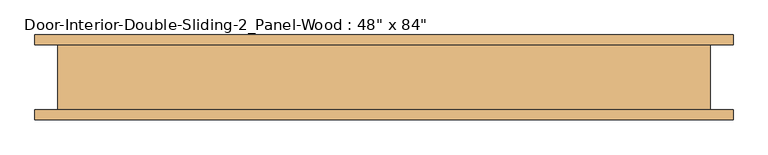
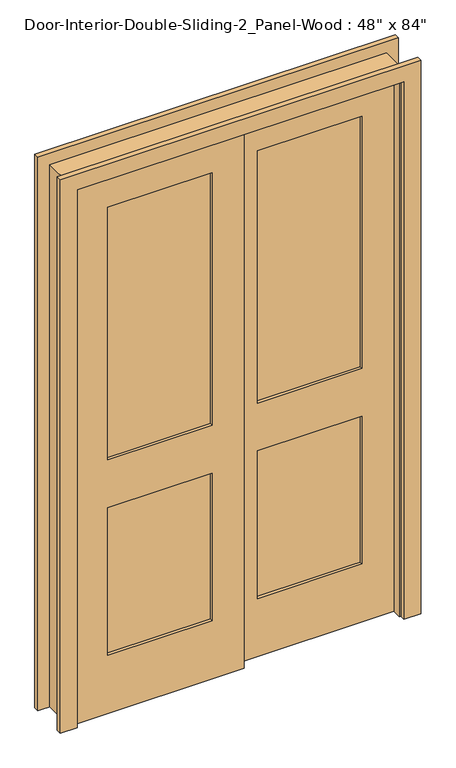
"""IFC4 building model written with IfcOpenShell, lengths in millimetres: door geometry."""

from ifc_helpers import new_model, si_unit, frame, origin, place, context, project, spatial, polyline, outline, extrude, source, transform, mapped, element, save


def door_39e6ccb1(model_context):
    return source(origin(), model_context, "Body", "SweptSolid", [
        extrude(outline(polyline([(488.95, -2.1166667), (488.95, -13.7583333), (95.25, -13.7583333), (95.25, -2.1166667), (488.95, -2.1166667)])), frame((0.0, 0.0, 1009.65), z_axis=(0.0, 0.0, 1.0), x_axis=(1.0, 0.0, 0.0)), (0.0, 0.0, 1.0), 1004.8875),
        extrude(outline(polyline([(488.95, -2.1166667), (488.95, -13.7583333), (95.25, -13.7583333), (95.25, -2.1166667), (488.95, -2.1166667)])), frame((0.0, 0.0, 231.775), z_axis=(0.0, 0.0, 1.0), x_axis=(1.0, 0.0, 0.0)), (0.0, 0.0, 1.0), 587.375),
        extrude(outline(polyline([(2133.6, -25.4), (0.0, -25.4), (0.0, 609.6), (2133.6, 609.6), (2133.6, -25.4)]), holes=[polyline([(2014.5375, 95.25), (2014.5375, 488.95), (1009.65, 488.95), (1009.65, 95.25), (2014.5375, 95.25)]), polyline([(819.15, 95.25), (819.15, 488.95), (231.775, 488.95), (231.775, 95.25), (819.15, 95.25)])]), frame((0.0, -25.4, 0.0), z_axis=(0.0, 1.0, 0.0), x_axis=(0.0, 0.0, 1.0)), (0.0, 0.0, 1.0), 34.925),
        extrude(outline(polyline([(-95.25, -37.0416667), (-95.25, -48.6833333), (-488.95, -48.6833333), (-488.95, -37.0416667), (-95.25, -37.0416667)])), frame((0.0, 0.0, 1009.65), z_axis=(0.0, 0.0, 1.0), x_axis=(1.0, 0.0, 0.0)), (0.0, 0.0, 1.0), 1004.8875),
        extrude(outline(polyline([(-95.25, -37.0416667), (-95.25, -48.6833333), (-488.95, -48.6833333), (-488.95, -37.0416667), (-95.25, -37.0416667)])), frame((0.0, 0.0, 231.775), z_axis=(0.0, 0.0, 1.0), x_axis=(1.0, 0.0, 0.0)), (0.0, 0.0, 1.0), 587.375),
        extrude(outline(polyline([(2133.6, -609.6), (0.0, -609.6), (0.0, 25.4), (2133.6, 25.4), (2133.6, -609.6)]), holes=[polyline([(2014.5375, -488.95), (2014.5375, -95.25), (1009.65, -95.25), (1009.65, -488.95), (2014.5375, -488.95)]), polyline([(819.15, -488.95), (819.15, -95.25), (231.775, -95.25), (231.775, -488.95), (819.15, -488.95)])]), frame((0.0, -60.325, 0.0), z_axis=(0.0, 1.0, 0.0), x_axis=(0.0, 0.0, 1.0)), (0.0, 0.0, 1.0), 34.925),
        extrude(outline(polyline([(0.0, 635.0), (2159.0, 635.0), (2159.0, -635.0), (0.0, -635.0), (0.0, -609.6), (2133.6, -609.6), (2133.6, 609.6), (0.0, 609.6), (0.0, 635.0)])), frame((0.0, -60.325, 0.0), z_axis=(0.0, 1.0, 0.0), x_axis=(0.0, 0.0, 1.0)), (0.0, 0.0, 1.0), 127.0),
        extrude(outline(polyline([(0.0, 679.45), (2203.45, 679.45), (2203.45, -679.45), (0.0, -679.45), (0.0, -615.95), (2139.95, -615.95), (2139.95, 615.95), (0.0, 615.95), (0.0, 679.45)])), frame((0.0, 66.675, 0.0), z_axis=(0.0, 1.0, 0.0), x_axis=(0.0, 0.0, 1.0)), (0.0, 0.0, 1.0), 19.05),
        extrude(outline(polyline([(0.0, 679.45), (2203.45, 679.45), (2203.45, -679.45), (0.0, -679.45), (0.0, -615.95), (2139.95, -615.95), (2139.95, 615.95), (0.0, 615.95), (0.0, 679.45)])), frame((0.0, -79.375, 0.0), z_axis=(0.0, 1.0, 0.0), x_axis=(0.0, 0.0, 1.0)), (0.0, 0.0, 1.0), 19.05),
    ])


if __name__ == "__main__":
    model = new_model("IFC4")
    model_context = context("Model", 3, world=origin())
    ifc_project = project(units=[si_unit("LENGTHUNIT", "METRE", prefix="MILLI")], contexts=[model_context])
    site = spatial("IfcSite", under=ifc_project)
    building = spatial("IfcBuilding", under=site)
    placement = place(None, origin())
    door_shape = door_39e6ccb1(model_context)
    element("IfcDoor", 1, ObjectType="Door-Interior-Double-Sliding-2_Panel-Wood : 48\" x 84\"", at=placement, inside=building, context=model_context, shape_type="MappedRepresentation", body=[
        mapped(door_shape, transform((0.0, 0.0, 0.0), x_axis=(1.0, 0.0, 0.0), y_axis=(0.0, 1.0, 0.0), z_axis=(0.0, 0.0, 1.0))),
    ])
    save(model, "model.ifc")

# Revit data of these elements
# Type "Door-Interior-Double-Sliding-2_Panel-Wood : 48\" x 84\""
#   Type Mark = "13"
#   Assembly Code = "C1020300"
#   Analytic Construction = "Wooden"
#   Top Rail = 0' - 4 11/16"
#   Thickness = 0' - 1 3/8"
#   Thermal Resistance (R) = 2.5876 (h·ft²·°F)/BTU
#   Stiles = 0' - 4 3/4"
#   Rough Width = 4' - 2"
#   Rough Height = 7' - 1"
#   Lock Rail = 0' - 7 1/2"
#   Height = 7' - 0"
#   Width = 4' - 0"
#   Heat Transfer Coefficient (U) = 0.3865 BTU/(h·ft²·°F)
#   Bottom Rail = 0' - 9 1/8"
#   Function = 0
#   Define Thermal Properties by = 1
#   Trim Material = Cherry
#   Panel Material = Cherry
#   Frame Material = Cherry
#   Visual Light Transmittance = 0
#   Solar Heat Gain Coefficient = 0
#   Wall Closure = (empty or 0)
#   Function = (empty or 0)
# Element 1 (IfcDoor, "Door-Interior-Double-Sliding-2_Panel-Wood : 48\" x 84\"")
#   Materials on its faces: "Cherry"
# Materials
#   "Cherry": class "Wood", colour RGB 157 77 38, transparency 0, Description = "Prunus Serotina", Cost = 0
